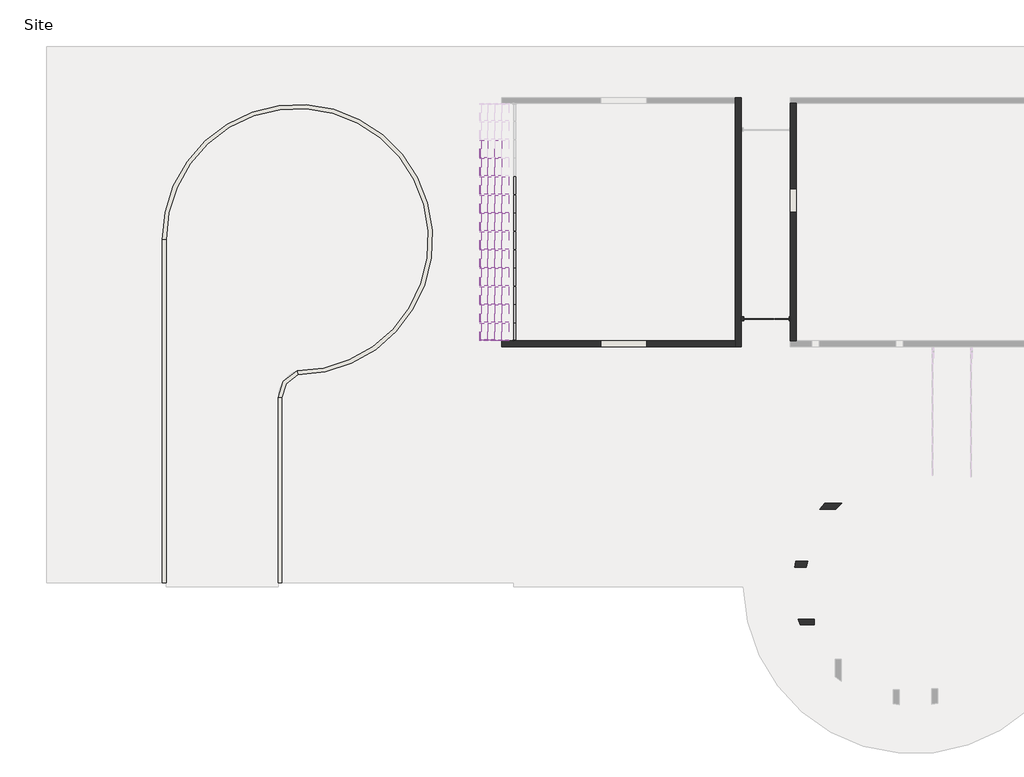
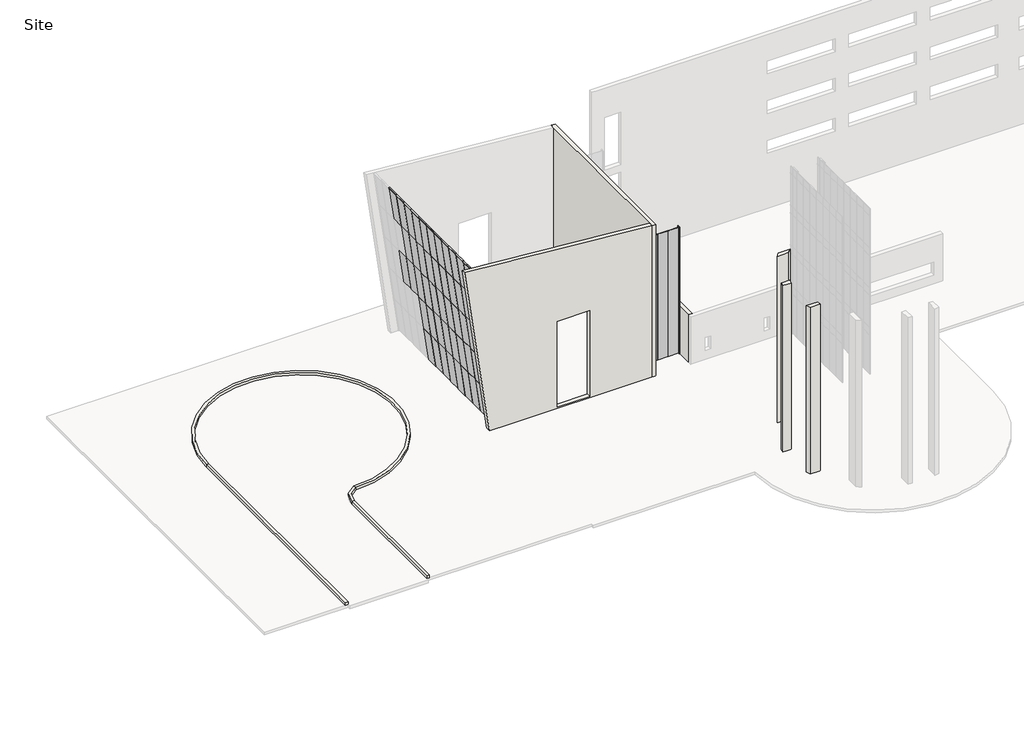
# One storey, part 1 of 4: 53 plates, 16 members, 12 walls.
"""IFC4 building model written with IfcOpenShell, lengths in millimetres."""

import ifcopenshell
import ifcopenshell.guid

model = None  # the IFC model being written
_history = None  # IfcOwnerHistory: only IFC2X3 demands one
_inside = {}  # id of a spatial element -> (the spatial element, [elements in it])
_under = {}  # id of a project, library or spatial element -> (it, [spatial elements below it])
_declared = {}  # id of a project -> (the project, [libraries it declares])
_typed = {}  # id of a type object -> (the type object, [elements of that type])
_made_of = {}  # id of a material, layer set ... -> (it, [elements and type objects made of it])


def new_model(schema):
    """Start an empty IFC model of exactly this schema.

    Asked for "IFC4X3", IfcOpenShell would pick the latest addendum, in which some entities
    have other attributes; the version numbers below select the first issue.
    IFC2X3 requires an IfcOwnerHistory on every rooted entity: one is made here for all.
    """
    global model, _history
    if schema == "IFC4X3":
        model = ifcopenshell.file(schema_version=(4, 3, 0, 0))
    else:
        model = ifcopenshell.file(schema=schema)
    _inside.clear()
    _under.clear()
    _declared.clear()
    _typed.clear()
    _made_of.clear()
    _history = None
    if model.schema == "IFC2X3":
        org = make("IfcOrganization", Name="unknown")
        user = make(
            "IfcPersonAndOrganization",
            ThePerson=make("IfcPerson", FamilyName="unknown"),
            TheOrganization=org,
        )
        app = make(
            "IfcApplication",
            ApplicationDeveloper=org,
            Version="unknown",
            ApplicationFullName="unknown",
            ApplicationIdentifier="unknown",
        )
        _history = make(
            "IfcOwnerHistory",
            OwningUser=user,
            OwningApplication=app,
            ChangeAction="ADDED",
            CreationDate=0,
        )
    return model


def make(cls, **values):
    """One entity of the class cls with the attributes given. An attribute that is None is left unset."""
    return model.create_entity(
        cls, **{name: value for name, value in values.items() if value is not None}
    )


def rooted(cls, **values):
    """An entity with a GlobalId (a new one), such as an element, a storey or a relation."""
    return make(cls, GlobalId=ifcopenshell.guid.new(), OwnerHistory=_history, **values)


def si_unit(unit_type, name, prefix=None):
    """IfcSIUnit, for example si_unit("LENGTHUNIT", "METRE", prefix="MILLI")."""
    return make("IfcSIUnit", UnitType=unit_type, Prefix=prefix, Name=name)


def assignment(units):
    """IfcUnitAssignment: the units of a project."""
    return None if units is None else make("IfcUnitAssignment", Units=units)


def point(xyz):
    """IfcCartesianPoint."""
    return None if xyz is None else make("IfcCartesianPoint", Coordinates=xyz)


def direction(xyz):
    """IfcDirection."""
    return None if xyz is None else make("IfcDirection", DirectionRatios=xyz)


def frame(location, z_axis=None, x_axis=None):
    """IfcAxis2Placement3D, a coordinate frame: its origin and axes. An axis left out is left unset."""
    return make(
        "IfcAxis2Placement3D",
        Location=point(location),
        Axis=direction(z_axis),
        RefDirection=direction(x_axis),
    )


def frame_2d(location, x_axis=None):
    """IfcAxis2Placement2D, a coordinate frame in the plane: its origin and x axis."""
    return make(
        "IfcAxis2Placement2D", Location=point(location), RefDirection=direction(x_axis)
    )


def origin():
    """The frame at (0, 0, 0) with its axes left unset."""
    return frame((0.0, 0.0, 0.0))


def origin_with_axes():
    """The frame at (0, 0, 0) with the z axis (0, 0, 1) and the x axis (1, 0, 0) written out."""
    return frame((0.0, 0.0, 0.0), z_axis=(0.0, 0.0, 1.0), x_axis=(1.0, 0.0, 0.0))


def place(relative_to, where):
    """IfcLocalPlacement: puts the frame where relative to a parent placement (None: the world)."""
    return make(
        "IfcLocalPlacement", PlacementRelTo=relative_to, RelativePlacement=where
    )


def context(
    kind, dimensions, precision=None, world=None, true_north=None, identifier=None
):
    """IfcGeometricRepresentationContext, for example the 3D "Model" context."""
    return make(
        "IfcGeometricRepresentationContext",
        ContextIdentifier=identifier,
        ContextType=kind,
        CoordinateSpaceDimension=dimensions,
        Precision=precision,
        WorldCoordinateSystem=world,
        TrueNorth=true_north,
    )


def project(units=None, contexts=None):
    """IfcProject with its units and contexts."""
    return rooted(
        "IfcProject",
        Name="project",
        RepresentationContexts=contexts,
        UnitsInContext=assignment(units),
    )


def spatial(cls, under=None, at=None, **own):
    """A site, building, storey or space (cls), placed at a placement, below another one or the project."""
    s = rooted(cls, ObjectPlacement=at, **own)
    if under is not None:
        _under.setdefault(under.id(), (under, []))[1].append(s)
    return s


def polyline(points):
    """IfcPolyline through the points."""
    return make("IfcPolyline", Points=[point(p) for p in points])


def circle_curve(where, radius):
    """IfcCircle in the frame where."""
    return make("IfcCircle", Position=where, Radius=radius)


def trimmed(basis, trim1, trim2, sense, master):
    """IfcTrimmedCurve: the piece of a basis curve between two trims."""
    return make(
        "IfcTrimmedCurve",
        BasisCurve=basis,
        Trim1=trim1,
        Trim2=trim2,
        SenseAgreement=sense,
        MasterRepresentation=master,
    )


def segment(curve, same_sense, transition):
    """IfcCompositeCurveSegment."""
    return make(
        "IfcCompositeCurveSegment",
        Transition=transition,
        SameSense=same_sense,
        ParentCurve=curve,
    )


def composite_curve(segments, self_intersect=None):
    """IfcCompositeCurve: segments joined end to end."""
    return make("IfcCompositeCurve", Segments=segments, SelfIntersect=self_intersect)


def outline(outer, holes=None, kind="AREA"):
    """IfcArbitraryClosedProfileDef: a profile drawn as a closed curve; with holes, ...WithVoids."""
    if holes is None:
        return make("IfcArbitraryClosedProfileDef", ProfileType=kind, OuterCurve=outer)
    return make(
        "IfcArbitraryProfileDefWithVoids",
        ProfileType=kind,
        OuterCurve=outer,
        InnerCurves=holes,
    )


def extrude(swept, where, along, depth):
    """IfcExtrudedAreaSolid: the profile swept, set in the frame where, extruded along a direction by depth."""
    return make(
        "IfcExtrudedAreaSolid",
        SweptArea=swept,
        Position=where,
        ExtrudedDirection=direction(along),
        Depth=depth,
    )


def faces_of(points, faces, orient=None, outer=None):
    """IfcFace entities. A face is a list of loops; a loop is a list of indices into points, from 0.

    orient and outer hold one flag for each loop. By default every Orientation is true, the
    first loop of a face is its IfcFaceOuterBound and the others are IfcFaceBound.
    """
    made = []
    for i, loops in enumerate(faces):
        bounds = []
        for j, loop in enumerate(loops):
            is_outer = j == 0 if outer is None else outer[i][j]
            bounds.append(
                make(
                    "IfcFaceOuterBound" if is_outer else "IfcFaceBound",
                    Bound=make("IfcPolyLoop", Polygon=[points[k] for k in loop]),
                    Orientation=True if orient is None else orient[i][j],
                )
            )
        made.append(make("IfcFace", Bounds=bounds))
    return made


def faceted_brep(points, faces, orient=None, outer=None, voids=None):
    """IfcFacetedBrep: a solid bounded by flat faces; with voids (closed shells), ...WithVoids."""
    shared = [point(p) for p in points]
    hull = make("IfcClosedShell", CfsFaces=faces_of(shared, faces, orient, outer))
    if voids is None:
        return make("IfcFacetedBrep", Outer=hull)
    return make(
        "IfcFacetedBrepWithVoids",
        Outer=hull,
        Voids=[
            make(cls, CfsFaces=faces_of(shared, fs, o, b)) for cls, fs, o, b in voids
        ],
    )


def shape(context_of_items, identifier, shape_type, items):
    """IfcShapeRepresentation: the items that make up one representation, for example the "Body"."""
    return make(
        "IfcShapeRepresentation",
        ContextOfItems=context_of_items,
        RepresentationIdentifier=identifier,
        RepresentationType=shape_type,
        Items=items,
    )


def source(mapping_origin, context_of_items, identifier, shape_type, items):
    """IfcRepresentationMap: a shape defined once, which mapped items show again and again."""
    return make(
        "IfcRepresentationMap",
        MappingOrigin=mapping_origin,
        MappedRepresentation=shape(context_of_items, identifier, shape_type, items),
    )


def transform(
    local_origin,
    x_axis=None,
    y_axis=None,
    z_axis=None,
    scale=None,
    scale2=None,
    scale3=None,
    uniform=True,
):
    """IfcCartesianTransformationOperator3D, or its non-uniform kind. x_axis, y_axis, z_axis: its Axis1, 2, 3."""
    if uniform:
        return make(
            "IfcCartesianTransformationOperator3D",
            Axis1=direction(x_axis),
            Axis2=direction(y_axis),
            LocalOrigin=point(local_origin),
            Scale=scale,
            Axis3=direction(z_axis),
        )
    return make(
        "IfcCartesianTransformationOperator3DnonUniform",
        Axis1=direction(x_axis),
        Axis2=direction(y_axis),
        LocalOrigin=point(local_origin),
        Scale=scale,
        Axis3=direction(z_axis),
        Scale2=scale2,
        Scale3=scale3,
    )


def mapped(mapping_source, mapping_target):
    """IfcMappedItem: shows the shape of a source again, moved by a transform."""
    return make(
        "IfcMappedItem", MappingSource=mapping_source, MappingTarget=mapping_target
    )


def made_of(thing, what):
    """Note that an element or type object is made of a material, layer set ...; save() writes the relation."""
    if what is not None:
        _made_of.setdefault(what.id(), (what, []))[1].append(thing)
    return thing


def element(
    cls,
    number,
    at=None,
    inside=None,
    cuts=None,
    type_object=None,
    material=None,
    context=None,
    identifier="Body",
    shape_type=None,
    held_by="IfcProductDefinitionShape",
    body=None,
    shapes=None,
    **own,
):
    """One element of the class cls, such as IfcWall. Its Tag is "e" and its number.

    at: its placement. inside: the storey or other place that contains it. cuts: it is an
    opening in that element (IfcRelVoidsElement). A single representation is given by context,
    identifier, shape_type and body (its items); several are given by shapes. held_by: the class
    of the entity that holds the representations. save() writes the other relations.
    """
    e = rooted(cls, Tag="e%d" % number, ObjectPlacement=at, **own)
    if body is not None:
        shapes = [shape(context, identifier, shape_type, body)]
    if shapes is not None:
        e.Representation = make(held_by, Representations=shapes)
    if inside is not None:
        _inside.setdefault(inside.id(), (inside, []))[1].append(e)
    if cuts is not None:
        rooted(
            "IfcRelVoidsElement", RelatingBuildingElement=cuts, RelatedOpeningElement=e
        )
    if type_object is not None:
        _typed.setdefault(type_object.id(), (type_object, []))[1].append(e)
    return made_of(e, material)


def aggregate(whole, parts):
    """IfcRelAggregates: a whole, such as a stair, and the parts it consists of."""
    return rooted("IfcRelAggregates", RelatingObject=whole, RelatedObjects=parts)


def save(model, path):
    """Write the relations noted so far, then the file.

    IfcRelAggregates (storeys below a building ...), IfcRelContainedInSpatialStructure (elements
    in a storey), IfcRelDefinesByType, IfcRelAssociatesMaterial and IfcRelDeclares: one each for
    every whole, place, type object, material and project.
    """
    for whole, parts in _under.values():
        aggregate(whole, parts)
    for where, things in _inside.values():
        rooted(
            "IfcRelContainedInSpatialStructure",
            RelatedElements=things,
            RelatingStructure=where,
        )
    for kind, things in _typed.values():
        rooted("IfcRelDefinesByType", RelatedObjects=things, RelatingType=kind)
    for what, things in _made_of.values():
        rooted("IfcRelAssociatesMaterial", RelatedObjects=things, RelatingMaterial=what)
    for by, libraries in _declared.values():
        rooted("IfcRelDeclares", RelatingContext=by, RelatedDefinitions=libraries)
    model.write(path)


def member_f8a9089e(model_context):
    return source(origin(), model_context, "Body", "SweptSolid", [
        extrude(outline(polyline([(0.0, 63.5), (0.0, -63.5), (-63.5, -63.5), (-63.5, 63.5), (0.0, 63.5)])), frame((0.0, 0.0, -1320.067308), z_axis=(0.0, 0.0, 1.0), x_axis=(1.0, 0.0, 0.0)), (0.0, 0.0, 1.0), 1320.067308),
    ])


def member_5e02c13a(model_context):
    return source(origin(), model_context, "Body", "SweptSolid", [
        extrude(outline(polyline([(0.0, 63.5), (0.0, -63.5), (-63.5, -63.5), (-63.5, 63.5), (0.0, 63.5)])), frame((0.0, 0.0, -1383.5673076), z_axis=(0.0, 0.0, 1.0), x_axis=(1.0, 0.0, 0.0)), (0.0, 0.0, 1.0), 1383.5673076),
    ])


def member_50cd645d(model_context):
    return source(origin(), model_context, "Body", "SweptSolid", [
        extrude(outline(polyline([(0.0, 63.5), (0.0, -63.5), (-63.5, -63.5), (-63.5, 63.5), (0.0, 63.5)])), frame((0.0, 0.0, -4003.5335741), z_axis=(0.0, 0.0, 1.0), x_axis=(1.0, 0.0, 0.0)), (0.0, 0.0, 1.0), 4003.5335741),
    ])


def member_5d333a65(model_context):
    return source(origin(), model_context, "Body", "SweptSolid", [
        extrude(outline(polyline([(0.0, 63.5), (0.0, -63.5), (-63.5, -63.5), (-63.5, 63.5), (0.0, 63.5)])), frame((0.0, 0.0, -3971.7835741), z_axis=(0.0, 0.0, 1.0), x_axis=(1.0, 0.0, 0.0)), (0.0, 0.0, 1.0), 3971.7835741),
    ])


def system_panel_glazed_21f2c726(model_context):
    return source(origin(), model_context, "Body", "SweptSolid", [
        extrude(outline(polyline([(553.4450969, 19.05), (-553.4450969, 19.05), (-553.4450969, 44.45), (553.4450969, 44.45), (553.4450969, 19.05)])), origin_with_axes(), (0.0, 0.0, 1.0), 14960.6),
    ])


def system_panel_glazed_1400d148(model_context):
    return source(origin(), model_context, "Body", "SweptSolid", [
        extrude(outline(polyline([(569.3200969, 19.05), (-569.3200969, 19.05), (-569.3200969, 44.45), (569.3200969, 44.45), (569.3200969, 19.05)])), origin_with_axes(), (0.0, 0.0, 1.0), 14960.6),
    ])


def system_panel_glazed_f91df05e(model_context):
    return source(origin(), model_context, "Body", "SweptSolid", [
        extrude(outline(polyline([(660.033654, 19.05), (-660.033654, 19.05), (-660.033654, 44.45), (660.033654, 44.45), (660.033654, 19.05)])), origin_with_axes(), (0.0, 0.0, 1.0), 3908.2835741),
    ])


def system_panel_glazed_78b5b18d(model_context):
    return source(origin(), model_context, "Body", "SweptSolid", [
        extrude(outline(polyline([(691.7836538, 19.05), (-691.7836538, 19.05), (-691.7836538, 44.45), (691.7836538, 44.45), (691.7836538, 19.05)])), origin_with_axes(), (0.0, 0.0, 1.0), 3908.2835741),
    ])


model = new_model("IFC4")

# Units and contexts
model_context = context("Model", 3, world=origin())
ifc_project = project(units=[si_unit("LENGTHUNIT", "METRE", prefix="MILLI")], contexts=[model_context])

# Site, building, storey
site = spatial("IfcSite", under=ifc_project)
building = spatial("IfcBuilding", under=site)
storey = spatial("IfcBuildingStorey", under=building, Name="Site", Elevation=-152.4)

# Members
placement = place(None, origin())
member_shape = member_f8a9089e(model_context)
element("IfcMember", 1, ObjectType="Rectangular Mullion1 : 2.5\" x 5\" rectangular", at=placement, inside=storey, context=model_context, shape_type="MappedRepresentation", body=[
    mapped(member_shape, transform((-27908.8595656, 38681.824389, 19574.3667708), x_axis=(-0.13917310096006533, 0.0, 0.9902680687415704), y_axis=(-0.9902680687415704, 0.0, -0.13917310096006533), z_axis=(0.0, -1.0, 0.0))),
])
member_2_shape = member_5e02c13a(model_context)
element("IfcMember", 2, ObjectType="Rectangular Mullion1 : 2.5\" x 5\" rectangular", at=placement, inside=storey, context=model_context, shape_type="MappedRepresentation", body=[
    mapped(member_2_shape, transform((-27908.8595656, 53088.9974658, 19574.3667708), x_axis=(-0.13917310096006533, 0.0, 0.9902680687415704), y_axis=(-0.9902680687415704, 0.0, -0.13917310096006533), z_axis=(0.0, -1.0, 0.0))),
])
element("IfcMember", 3, ObjectType="Rectangular Mullion1 : 2.5\" x 5\" rectangular", at=placement, inside=storey, context=model_context, shape_type="MappedRepresentation", body=[
    mapped(member_2_shape, transform((-27908.8595656, 51641.9301581, 19574.3667708), x_axis=(-0.13917310096006533, 0.0, 0.9902680687415704), y_axis=(-0.9902680687415704, 0.0, -0.13917310096006533), z_axis=(0.0, -1.0, 0.0))),
])
element("IfcMember", 4, ObjectType="Rectangular Mullion1 : 2.5\" x 5\" rectangular", at=placement, inside=storey, context=model_context, shape_type="MappedRepresentation", body=[
    mapped(member_2_shape, transform((-27908.8595656, 50194.8628505, 19574.3667708), x_axis=(-0.13917310096006533, 0.0, 0.9902680687415704), y_axis=(-0.9902680687415704, 0.0, -0.13917310096006533), z_axis=(0.0, -1.0, 0.0))),
])
element("IfcMember", 5, ObjectType="Rectangular Mullion1 : 2.5\" x 5\" rectangular", at=placement, inside=storey, context=model_context, shape_type="MappedRepresentation", body=[
    mapped(member_2_shape, transform((-27908.8595656, 48747.7955428, 19574.3667708), x_axis=(-0.13917310096006533, 0.0, 0.9902680687415704), y_axis=(-0.9902680687415704, 0.0, -0.13917310096006533), z_axis=(0.0, -1.0, 0.0))),
])
element("IfcMember", 6, ObjectType="Rectangular Mullion1 : 2.5\" x 5\" rectangular", at=placement, inside=storey, context=model_context, shape_type="MappedRepresentation", body=[
    mapped(member_2_shape, transform((-27908.8595656, 47300.7282352, 19574.3667708), x_axis=(-0.13917310096006533, 0.0, 0.9902680687415704), y_axis=(-0.9902680687415704, 0.0, -0.13917310096006533), z_axis=(0.0, -1.0, 0.0))),
])
element("IfcMember", 7, ObjectType="Rectangular Mullion1 : 2.5\" x 5\" rectangular", at=placement, inside=storey, context=model_context, shape_type="MappedRepresentation", body=[
    mapped(member_2_shape, transform((-27908.8595656, 45853.6609275, 19574.3667708), x_axis=(-0.13917310096006533, 0.0, 0.9902680687415704), y_axis=(-0.9902680687415704, 0.0, -0.13917310096006533), z_axis=(0.0, -1.0, 0.0))),
])
element("IfcMember", 8, ObjectType="Rectangular Mullion1 : 2.5\" x 5\" rectangular", at=placement, inside=storey, context=model_context, shape_type="MappedRepresentation", body=[
    mapped(member_2_shape, transform((-27908.8595656, 44406.5936199, 19574.3667708), x_axis=(-0.13917310096006533, 0.0, 0.9902680687415704), y_axis=(-0.9902680687415704, 0.0, -0.13917310096006533), z_axis=(0.0, -1.0, 0.0))),
])
element("IfcMember", 9, ObjectType="Rectangular Mullion1 : 2.5\" x 5\" rectangular", at=placement, inside=storey, context=model_context, shape_type="MappedRepresentation", body=[
    mapped(member_2_shape, transform((-27908.8595656, 42959.5263122, 19574.3667708), x_axis=(-0.13917310096006533, 0.0, 0.9902680687415704), y_axis=(-0.9902680687415704, 0.0, -0.13917310096006533), z_axis=(0.0, -1.0, 0.0))),
])
element("IfcMember", 10, ObjectType="Rectangular Mullion1 : 2.5\" x 5\" rectangular", at=placement, inside=storey, context=model_context, shape_type="MappedRepresentation", body=[
    mapped(member_2_shape, transform((-27908.8595656, 41512.4590046, 19574.3667708), x_axis=(-0.13917310096006533, 0.0, 0.9902680687415704), y_axis=(-0.9902680687415704, 0.0, -0.13917310096006533), z_axis=(0.0, -1.0, 0.0))),
])
element("IfcMember", 11, ObjectType="Rectangular Mullion1 : 2.5\" x 5\" rectangular", at=placement, inside=storey, context=model_context, shape_type="MappedRepresentation", body=[
    mapped(member_2_shape, transform((-27908.8595656, 40065.391697, 19574.3667708), x_axis=(-0.13917310096006533, 0.0, 0.9902680687415704), y_axis=(-0.9902680687415704, 0.0, -0.13917310096006533), z_axis=(0.0, -1.0, 0.0))),
])
member_3_shape = member_50cd645d(model_context)
element("IfcMember", 12, ObjectType="Rectangular Mullion1 : 2.5\" x 5\" rectangular", at=placement, inside=storey, context=model_context, shape_type="MappedRepresentation", body=[
    mapped(member_3_shape, transform((-25136.1948919, 38618.324389, -154.1674984), x_axis=(0.0, -1.0, 0.0), y_axis=(-0.99026806874157, 0.0, -0.1391731009600678), z_axis=(0.1391731009600678, 0.0, -0.99026806874157))),
])
member_4_shape = member_5d333a65(model_context)
element("IfcMember", 13, ObjectType="Rectangular Mullion1 : 2.5\" x 5\" rectangular", at=placement, inside=storey, context=model_context, shape_type="MappedRepresentation", body=[
    mapped(member_4_shape, transform((-25693.3790742, 38618.324389, 3810.4039622), x_axis=(0.0, -1.0, 0.0), y_axis=(-0.9902680687415704, 0.0, -0.13917310096006566), z_axis=(0.13917310096006566, 0.0, -0.9902680687415704))),
])
element("IfcMember", 14, ObjectType="Rectangular Mullion1 : 2.5\" x 5\" rectangular", at=placement, inside=storey, context=model_context, shape_type="MappedRepresentation", body=[
    mapped(member_4_shape, transform((-26246.1445106, 38618.324389, 7743.5344115), x_axis=(0.0, -1.0, 0.0), y_axis=(-0.9902680687415704, 0.0, -0.13917310096006574), z_axis=(0.13917310096006574, 0.0, -0.9902680687415704))),
])
element("IfcMember", 15, ObjectType="Rectangular Mullion1 : 2.5\" x 5\" rectangular", at=placement, inside=storey, context=model_context, shape_type="MappedRepresentation", body=[
    mapped(member_4_shape, transform((-26798.9099469, 38618.324389, 11676.6648609), x_axis=(0.0, -1.0, 0.0), y_axis=(-0.9902680687415705, 0.0, -0.13917310096006458), z_axis=(0.13917310096006458, 0.0, -0.9902680687415705))),
])
element("IfcMember", 16, ObjectType="Rectangular Mullion1 : 2.5\" x 5\" rectangular", at=placement, inside=storey, context=model_context, shape_type="MappedRepresentation", body=[
    mapped(member_3_shape, transform((-27351.6753833, 38618.324389, 15609.7953102), x_axis=(0.0, -1.0, 0.0), y_axis=(-0.9902680687415704, 0.0, -0.13917310096006558), z_axis=(0.13917310096006558, 0.0, -0.9902680687415704))),
])

# Plates
system_panel_glazed_shape = system_panel_glazed_21f2c726(model_context)
element("IfcPlate", 17, ObjectType="System Panel : Glazed", at=placement, inside=storey, context=model_context, shape_type="MappedRepresentation", body=[
    mapped(system_panel_glazed_shape, transform((-4114.5553134, 40372.511889, -88.9), x_axis=(-1.0, 0.0, 0.0), y_axis=(0.0, -1.0, 0.0), z_axis=(0.0, 0.0, 1.0))),
])
element("IfcPlate", 18, ObjectType="System Panel : Glazed", at=placement, inside=storey, context=model_context, shape_type="MappedRepresentation", body=[
    mapped(system_panel_glazed_shape, transform((-6487.0857008, 40372.511889, -88.9), x_axis=(-1.0, 0.0, 0.0), y_axis=(0.0, -1.0, 0.0), z_axis=(0.0, 0.0, 1.0))),
])
system_panel_glazed_2_shape = system_panel_glazed_1400d148(model_context)
element("IfcPlate", 19, ObjectType="System Panel : Glazed", at=placement, inside=storey, context=model_context, shape_type="MappedRepresentation", body=[
    mapped(system_panel_glazed_2_shape, transform((-5300.8205071, 40372.511889, -88.9), x_axis=(-1.0, 0.0, 0.0), y_axis=(0.0, -1.0, 0.0), z_axis=(0.0, 0.0, 1.0))),
])
system_panel_glazed_3_shape = system_panel_glazed_f91df05e(model_context)
element("IfcPlate", 20, ObjectType="System Panel : Glazed", at=placement, inside=storey, context=model_context, shape_type="MappedRepresentation", body=[
    mapped(system_panel_glazed_3_shape, transform((-25145.0323838, 39341.858043, -91.285476), x_axis=(0.0, -1.0, 0.0), y_axis=(0.9902680687415704, 0.0, 0.13917310096006547), z_axis=(-0.13917310096006547, 0.0, 0.9902680687415704))),
])
element("IfcPlate", 21, ObjectType="System Panel : Glazed", at=placement, inside=storey, context=model_context, shape_type="MappedRepresentation", body=[
    mapped(system_panel_glazed_3_shape, transform((-25697.7978202, 39341.858043, 3841.8449733), x_axis=(0.0, -1.0, 0.0), y_axis=(0.9902680687415704, 0.0, 0.13917310096006533), z_axis=(-0.13917310096006533, 0.0, 0.9902680687415704))),
])
element("IfcPlate", 22, ObjectType="System Panel : Glazed", at=placement, inside=storey, context=model_context, shape_type="MappedRepresentation", body=[
    mapped(system_panel_glazed_3_shape, transform((-26250.5632565, 39341.858043, 7774.9754227), x_axis=(0.0, -1.0, 0.0), y_axis=(0.9902680687415704, 0.0, 0.13917310096006533), z_axis=(-0.13917310096006533, 0.0, 0.9902680687415704))),
])
element("IfcPlate", 23, ObjectType="System Panel : Glazed", at=placement, inside=storey, context=model_context, shape_type="MappedRepresentation", body=[
    mapped(system_panel_glazed_3_shape, transform((-26803.3286929, 39341.858043, 11708.105872), x_axis=(0.0, -1.0, 0.0), y_axis=(0.9902680687415704, 0.0, 0.13917310096006533), z_axis=(-0.13917310096006533, 0.0, 0.9902680687415704))),
])
element("IfcPlate", 24, ObjectType="System Panel : Glazed", at=placement, inside=storey, context=model_context, shape_type="MappedRepresentation", body=[
    mapped(system_panel_glazed_3_shape, transform((-27356.0941292, 39341.858043, 15641.2363214), x_axis=(0.0, -1.0, 0.0), y_axis=(0.9902680687415704, 0.0, 0.13917310096006533), z_axis=(-0.13917310096006533, 0.0, 0.9902680687415704))),
])
system_panel_glazed_4_shape = system_panel_glazed_78b5b18d(model_context)
element("IfcPlate", 25, ObjectType="System Panel : Glazed", at=placement, inside=storey, context=model_context, shape_type="MappedRepresentation", body=[
    mapped(system_panel_glazed_4_shape, transform((-25145.0323838, 50886.6465043, -91.285476), x_axis=(0.0, -1.0, 0.0), y_axis=(0.9902680687415704, 0.0, 0.13917310096006547), z_axis=(-0.13917310096006547, 0.0, 0.9902680687415704))),
])
element("IfcPlate", 26, ObjectType="System Panel : Glazed", at=placement, inside=storey, context=model_context, shape_type="MappedRepresentation", body=[
    mapped(system_panel_glazed_4_shape, transform((-25145.0323838, 49439.5791967, -91.285476), x_axis=(0.0, -1.0, 0.0), y_axis=(0.9902680687415704, 0.0, 0.13917310096006547), z_axis=(-0.13917310096006547, 0.0, 0.9902680687415704))),
])
element("IfcPlate", 27, ObjectType="System Panel : Glazed", at=placement, inside=storey, context=model_context, shape_type="MappedRepresentation", body=[
    mapped(system_panel_glazed_4_shape, transform((-25145.0323838, 47992.511889, -91.285476), x_axis=(0.0, -1.0, 0.0), y_axis=(0.9902680687415704, 0.0, 0.13917310096006547), z_axis=(-0.13917310096006547, 0.0, 0.9902680687415704))),
])
element("IfcPlate", 28, ObjectType="System Panel : Glazed", at=placement, inside=storey, context=model_context, shape_type="MappedRepresentation", body=[
    mapped(system_panel_glazed_4_shape, transform((-25145.0323838, 46545.4445814, -91.285476), x_axis=(0.0, -1.0, 0.0), y_axis=(0.9902680687415704, 0.0, 0.13917310096006547), z_axis=(-0.13917310096006547, 0.0, 0.9902680687415704))),
])
element("IfcPlate", 29, ObjectType="System Panel : Glazed", at=placement, inside=storey, context=model_context, shape_type="MappedRepresentation", body=[
    mapped(system_panel_glazed_4_shape, transform((-25145.0323838, 45098.3772737, -91.285476), x_axis=(0.0, -1.0, 0.0), y_axis=(0.9902680687415704, 0.0, 0.13917310096006547), z_axis=(-0.13917310096006547, 0.0, 0.9902680687415704))),
])
element("IfcPlate", 30, ObjectType="System Panel : Glazed", at=placement, inside=storey, context=model_context, shape_type="MappedRepresentation", body=[
    mapped(system_panel_glazed_4_shape, transform((-25145.0323838, 43651.3099661, -91.285476), x_axis=(0.0, -1.0, 0.0), y_axis=(0.9902680687415704, 0.0, 0.13917310096006547), z_axis=(-0.13917310096006547, 0.0, 0.9902680687415704))),
])
element("IfcPlate", 31, ObjectType="System Panel : Glazed", at=placement, inside=storey, context=model_context, shape_type="MappedRepresentation", body=[
    mapped(system_panel_glazed_4_shape, transform((-25145.0323838, 42204.2426584, -91.285476), x_axis=(0.0, -1.0, 0.0), y_axis=(0.9902680687415704, 0.0, 0.13917310096006547), z_axis=(-0.13917310096006547, 0.0, 0.9902680687415704))),
])
element("IfcPlate", 32, ObjectType="System Panel : Glazed", at=placement, inside=storey, context=model_context, shape_type="MappedRepresentation", body=[
    mapped(system_panel_glazed_4_shape, transform((-25145.0323838, 40757.1753508, -91.285476), x_axis=(0.0, -1.0, 0.0), y_axis=(0.9902680687415704, 0.0, 0.13917310096006547), z_axis=(-0.13917310096006547, 0.0, 0.9902680687415704))),
])
element("IfcPlate", 33, ObjectType="System Panel : Glazed", at=placement, inside=storey, context=model_context, shape_type="MappedRepresentation", body=[
    mapped(system_panel_glazed_4_shape, transform((-25697.7978202, 50886.6465043, 3841.8449733), x_axis=(0.0, -1.0, 0.0), y_axis=(0.9902680687415704, 0.0, 0.13917310096006533), z_axis=(-0.13917310096006533, 0.0, 0.9902680687415704))),
])
element("IfcPlate", 34, ObjectType="System Panel : Glazed", at=placement, inside=storey, context=model_context, shape_type="MappedRepresentation", body=[
    mapped(system_panel_glazed_4_shape, transform((-25697.7978202, 49439.5791967, 3841.8449733), x_axis=(0.0, -1.0, 0.0), y_axis=(0.9902680687415704, 0.0, 0.13917310096006533), z_axis=(-0.13917310096006533, 0.0, 0.9902680687415704))),
])
element("IfcPlate", 35, ObjectType="System Panel : Glazed", at=placement, inside=storey, context=model_context, shape_type="MappedRepresentation", body=[
    mapped(system_panel_glazed_4_shape, transform((-25697.7978202, 47992.511889, 3841.8449733), x_axis=(0.0, -1.0, 0.0), y_axis=(0.9902680687415704, 0.0, 0.13917310096006533), z_axis=(-0.13917310096006533, 0.0, 0.9902680687415704))),
])
element("IfcPlate", 36, ObjectType="System Panel : Glazed", at=placement, inside=storey, context=model_context, shape_type="MappedRepresentation", body=[
    mapped(system_panel_glazed_4_shape, transform((-25697.7978202, 46545.4445814, 3841.8449733), x_axis=(0.0, -1.0, 0.0), y_axis=(0.9902680687415704, 0.0, 0.13917310096006533), z_axis=(-0.13917310096006533, 0.0, 0.9902680687415704))),
])
element("IfcPlate", 37, ObjectType="System Panel : Glazed", at=placement, inside=storey, context=model_context, shape_type="MappedRepresentation", body=[
    mapped(system_panel_glazed_4_shape, transform((-25697.7978202, 45098.3772737, 3841.8449733), x_axis=(0.0, -1.0, 0.0), y_axis=(0.9902680687415704, 0.0, 0.13917310096006533), z_axis=(-0.13917310096006533, 0.0, 0.9902680687415704))),
])
element("IfcPlate", 38, ObjectType="System Panel : Glazed", at=placement, inside=storey, context=model_context, shape_type="MappedRepresentation", body=[
    mapped(system_panel_glazed_4_shape, transform((-25697.7978202, 43651.3099661, 3841.8449733), x_axis=(0.0, -1.0, 0.0), y_axis=(0.9902680687415704, 0.0, 0.13917310096006533), z_axis=(-0.13917310096006533, 0.0, 0.9902680687415704))),
])
element("IfcPlate", 39, ObjectType="System Panel : Glazed", at=placement, inside=storey, context=model_context, shape_type="MappedRepresentation", body=[
    mapped(system_panel_glazed_4_shape, transform((-25697.7978202, 42204.2426584, 3841.8449733), x_axis=(0.0, -1.0, 0.0), y_axis=(0.9902680687415704, 0.0, 0.13917310096006533), z_axis=(-0.13917310096006533, 0.0, 0.9902680687415704))),
])
element("IfcPlate", 40, ObjectType="System Panel : Glazed", at=placement, inside=storey, context=model_context, shape_type="MappedRepresentation", body=[
    mapped(system_panel_glazed_4_shape, transform((-25697.7978202, 40757.1753508, 3841.8449733), x_axis=(0.0, -1.0, 0.0), y_axis=(0.9902680687415704, 0.0, 0.13917310096006533), z_axis=(-0.13917310096006533, 0.0, 0.9902680687415704))),
])
element("IfcPlate", 41, ObjectType="System Panel : Glazed", at=placement, inside=storey, context=model_context, shape_type="MappedRepresentation", body=[
    mapped(system_panel_glazed_4_shape, transform((-26250.5632565, 53780.7811196, 7774.9754227), x_axis=(0.0, -1.0, 0.0), y_axis=(0.9902680687415704, 0.0, 0.13917310096006533), z_axis=(-0.13917310096006533, 0.0, 0.9902680687415704))),
])
element("IfcPlate", 42, ObjectType="System Panel : Glazed", at=placement, inside=storey, context=model_context, shape_type="MappedRepresentation", body=[
    mapped(system_panel_glazed_4_shape, transform((-26250.5632565, 52333.7138119, 7774.9754227), x_axis=(0.0, -1.0, 0.0), y_axis=(0.9902680687415704, 0.0, 0.13917310096006533), z_axis=(-0.13917310096006533, 0.0, 0.9902680687415704))),
])
element("IfcPlate", 43, ObjectType="System Panel : Glazed", at=placement, inside=storey, context=model_context, shape_type="MappedRepresentation", body=[
    mapped(system_panel_glazed_4_shape, transform((-26250.5632565, 50886.6465043, 7774.9754227), x_axis=(0.0, -1.0, 0.0), y_axis=(0.9902680687415704, 0.0, 0.13917310096006533), z_axis=(-0.13917310096006533, 0.0, 0.9902680687415704))),
])
element("IfcPlate", 44, ObjectType="System Panel : Glazed", at=placement, inside=storey, context=model_context, shape_type="MappedRepresentation", body=[
    mapped(system_panel_glazed_4_shape, transform((-26250.5632565, 49439.5791967, 7774.9754227), x_axis=(0.0, -1.0, 0.0), y_axis=(0.9902680687415704, 0.0, 0.13917310096006533), z_axis=(-0.13917310096006533, 0.0, 0.9902680687415704))),
])
element("IfcPlate", 45, ObjectType="System Panel : Glazed", at=placement, inside=storey, context=model_context, shape_type="MappedRepresentation", body=[
    mapped(system_panel_glazed_4_shape, transform((-26250.5632565, 47992.511889, 7774.9754227), x_axis=(0.0, -1.0, 0.0), y_axis=(0.9902680687415704, 0.0, 0.13917310096006533), z_axis=(-0.13917310096006533, 0.0, 0.9902680687415704))),
])
element("IfcPlate", 46, ObjectType="System Panel : Glazed", at=placement, inside=storey, context=model_context, shape_type="MappedRepresentation", body=[
    mapped(system_panel_glazed_4_shape, transform((-26250.5632565, 46545.4445814, 7774.9754227), x_axis=(0.0, -1.0, 0.0), y_axis=(0.9902680687415704, 0.0, 0.13917310096006533), z_axis=(-0.13917310096006533, 0.0, 0.9902680687415704))),
])
element("IfcPlate", 47, ObjectType="System Panel : Glazed", at=placement, inside=storey, context=model_context, shape_type="MappedRepresentation", body=[
    mapped(system_panel_glazed_4_shape, transform((-26250.5632565, 45098.3772737, 7774.9754227), x_axis=(0.0, -1.0, 0.0), y_axis=(0.9902680687415704, 0.0, 0.13917310096006533), z_axis=(-0.13917310096006533, 0.0, 0.9902680687415704))),
])
element("IfcPlate", 48, ObjectType="System Panel : Glazed", at=placement, inside=storey, context=model_context, shape_type="MappedRepresentation", body=[
    mapped(system_panel_glazed_4_shape, transform((-26250.5632565, 43651.3099661, 7774.9754227), x_axis=(0.0, -1.0, 0.0), y_axis=(0.9902680687415704, 0.0, 0.13917310096006533), z_axis=(-0.13917310096006533, 0.0, 0.9902680687415704))),
])
element("IfcPlate", 49, ObjectType="System Panel : Glazed", at=placement, inside=storey, context=model_context, shape_type="MappedRepresentation", body=[
    mapped(system_panel_glazed_4_shape, transform((-26250.5632565, 42204.2426584, 7774.9754227), x_axis=(0.0, -1.0, 0.0), y_axis=(0.9902680687415704, 0.0, 0.13917310096006533), z_axis=(-0.13917310096006533, 0.0, 0.9902680687415704))),
])
element("IfcPlate", 50, ObjectType="System Panel : Glazed", at=placement, inside=storey, context=model_context, shape_type="MappedRepresentation", body=[
    mapped(system_panel_glazed_4_shape, transform((-26250.5632565, 40757.1753508, 7774.9754227), x_axis=(0.0, -1.0, 0.0), y_axis=(0.9902680687415704, 0.0, 0.13917310096006533), z_axis=(-0.13917310096006533, 0.0, 0.9902680687415704))),
])
element("IfcPlate", 51, ObjectType="System Panel : Glazed", at=placement, inside=storey, context=model_context, shape_type="MappedRepresentation", body=[
    mapped(system_panel_glazed_4_shape, transform((-26803.3286929, 52333.7138119, 11708.105872), x_axis=(0.0, -1.0, 0.0), y_axis=(0.9902680687415704, 0.0, 0.13917310096006533), z_axis=(-0.13917310096006533, 0.0, 0.9902680687415704))),
])
element("IfcPlate", 52, ObjectType="System Panel : Glazed", at=placement, inside=storey, context=model_context, shape_type="MappedRepresentation", body=[
    mapped(system_panel_glazed_4_shape, transform((-26803.3286929, 50886.6465043, 11708.105872), x_axis=(0.0, -1.0, 0.0), y_axis=(0.9902680687415704, 0.0, 0.13917310096006533), z_axis=(-0.13917310096006533, 0.0, 0.9902680687415704))),
])
element("IfcPlate", 53, ObjectType="System Panel : Glazed", at=placement, inside=storey, context=model_context, shape_type="MappedRepresentation", body=[
    mapped(system_panel_glazed_4_shape, transform((-26803.3286929, 49439.5791967, 11708.105872), x_axis=(0.0, -1.0, 0.0), y_axis=(0.9902680687415704, 0.0, 0.13917310096006533), z_axis=(-0.13917310096006533, 0.0, 0.9902680687415704))),
])
element("IfcPlate", 54, ObjectType="System Panel : Glazed", at=placement, inside=storey, context=model_context, shape_type="MappedRepresentation", body=[
    mapped(system_panel_glazed_4_shape, transform((-26803.3286929, 47992.511889, 11708.105872), x_axis=(0.0, -1.0, 0.0), y_axis=(0.9902680687415704, 0.0, 0.13917310096006533), z_axis=(-0.13917310096006533, 0.0, 0.9902680687415704))),
])
element("IfcPlate", 55, ObjectType="System Panel : Glazed", at=placement, inside=storey, context=model_context, shape_type="MappedRepresentation", body=[
    mapped(system_panel_glazed_4_shape, transform((-26803.3286929, 46545.4445814, 11708.105872), x_axis=(0.0, -1.0, 0.0), y_axis=(0.9902680687415704, 0.0, 0.13917310096006533), z_axis=(-0.13917310096006533, 0.0, 0.9902680687415704))),
])
element("IfcPlate", 56, ObjectType="System Panel : Glazed", at=placement, inside=storey, context=model_context, shape_type="MappedRepresentation", body=[
    mapped(system_panel_glazed_4_shape, transform((-26803.3286929, 45098.3772737, 11708.105872), x_axis=(0.0, -1.0, 0.0), y_axis=(0.9902680687415704, 0.0, 0.13917310096006533), z_axis=(-0.13917310096006533, 0.0, 0.9902680687415704))),
])
element("IfcPlate", 57, ObjectType="System Panel : Glazed", at=placement, inside=storey, context=model_context, shape_type="MappedRepresentation", body=[
    mapped(system_panel_glazed_4_shape, transform((-26803.3286929, 43651.3099661, 11708.105872), x_axis=(0.0, -1.0, 0.0), y_axis=(0.9902680687415704, 0.0, 0.13917310096006533), z_axis=(-0.13917310096006533, 0.0, 0.9902680687415704))),
])
element("IfcPlate", 58, ObjectType="System Panel : Glazed", at=placement, inside=storey, context=model_context, shape_type="MappedRepresentation", body=[
    mapped(system_panel_glazed_4_shape, transform((-26803.3286929, 42204.2426584, 11708.105872), x_axis=(0.0, -1.0, 0.0), y_axis=(0.9902680687415704, 0.0, 0.13917310096006533), z_axis=(-0.13917310096006533, 0.0, 0.9902680687415704))),
])
element("IfcPlate", 59, ObjectType="System Panel : Glazed", at=placement, inside=storey, context=model_context, shape_type="MappedRepresentation", body=[
    mapped(system_panel_glazed_4_shape, transform((-26803.3286929, 40757.1753508, 11708.105872), x_axis=(0.0, -1.0, 0.0), y_axis=(0.9902680687415704, 0.0, 0.13917310096006533), z_axis=(-0.13917310096006533, 0.0, 0.9902680687415704))),
])
element("IfcPlate", 60, ObjectType="System Panel : Glazed", at=placement, inside=storey, context=model_context, shape_type="MappedRepresentation", body=[
    mapped(system_panel_glazed_4_shape, transform((-27356.0941292, 53780.7811196, 15641.2363214), x_axis=(0.0, -1.0, 0.0), y_axis=(0.9902680687415704, 0.0, 0.13917310096006533), z_axis=(-0.13917310096006533, 0.0, 0.9902680687415704))),
])
element("IfcPlate", 61, ObjectType="System Panel : Glazed", at=placement, inside=storey, context=model_context, shape_type="MappedRepresentation", body=[
    mapped(system_panel_glazed_4_shape, transform((-27356.0941292, 52333.7138119, 15641.2363214), x_axis=(0.0, -1.0, 0.0), y_axis=(0.9902680687415704, 0.0, 0.13917310096006533), z_axis=(-0.13917310096006533, 0.0, 0.9902680687415704))),
])
element("IfcPlate", 62, ObjectType="System Panel : Glazed", at=placement, inside=storey, context=model_context, shape_type="MappedRepresentation", body=[
    mapped(system_panel_glazed_4_shape, transform((-27356.0941292, 50886.6465043, 15641.2363214), x_axis=(0.0, -1.0, 0.0), y_axis=(0.9902680687415704, 0.0, 0.13917310096006533), z_axis=(-0.13917310096006533, 0.0, 0.9902680687415704))),
])
element("IfcPlate", 63, ObjectType="System Panel : Glazed", at=placement, inside=storey, context=model_context, shape_type="MappedRepresentation", body=[
    mapped(system_panel_glazed_4_shape, transform((-27356.0941292, 49439.5791967, 15641.2363214), x_axis=(0.0, -1.0, 0.0), y_axis=(0.9902680687415704, 0.0, 0.13917310096006533), z_axis=(-0.13917310096006533, 0.0, 0.9902680687415704))),
])
element("IfcPlate", 64, ObjectType="System Panel : Glazed", at=placement, inside=storey, context=model_context, shape_type="MappedRepresentation", body=[
    mapped(system_panel_glazed_4_shape, transform((-27356.0941292, 47992.511889, 15641.2363214), x_axis=(0.0, -1.0, 0.0), y_axis=(0.9902680687415704, 0.0, 0.13917310096006533), z_axis=(-0.13917310096006533, 0.0, 0.9902680687415704))),
])
element("IfcPlate", 65, ObjectType="System Panel : Glazed", at=placement, inside=storey, context=model_context, shape_type="MappedRepresentation", body=[
    mapped(system_panel_glazed_4_shape, transform((-27356.0941292, 46545.4445814, 15641.2363214), x_axis=(0.0, -1.0, 0.0), y_axis=(0.9902680687415704, 0.0, 0.13917310096006533), z_axis=(-0.13917310096006533, 0.0, 0.9902680687415704))),
])
element("IfcPlate", 66, ObjectType="System Panel : Glazed", at=placement, inside=storey, context=model_context, shape_type="MappedRepresentation", body=[
    mapped(system_panel_glazed_4_shape, transform((-27356.0941292, 45098.3772737, 15641.2363214), x_axis=(0.0, -1.0, 0.0), y_axis=(0.9902680687415704, 0.0, 0.13917310096006533), z_axis=(-0.13917310096006533, 0.0, 0.9902680687415704))),
])
element("IfcPlate", 67, ObjectType="System Panel : Glazed", at=placement, inside=storey, context=model_context, shape_type="MappedRepresentation", body=[
    mapped(system_panel_glazed_4_shape, transform((-27356.0941292, 43651.3099661, 15641.2363214), x_axis=(0.0, -1.0, 0.0), y_axis=(0.9902680687415704, 0.0, 0.13917310096006533), z_axis=(-0.13917310096006533, 0.0, 0.9902680687415704))),
])
element("IfcPlate", 68, ObjectType="System Panel : Glazed", at=placement, inside=storey, context=model_context, shape_type="MappedRepresentation", body=[
    mapped(system_panel_glazed_4_shape, transform((-27356.0941292, 42204.2426584, 15641.2363214), x_axis=(0.0, -1.0, 0.0), y_axis=(0.9902680687415704, 0.0, 0.13917310096006533), z_axis=(-0.13917310096006533, 0.0, 0.9902680687415704))),
])
element("IfcPlate", 69, ObjectType="System Panel : Glazed", at=placement, inside=storey, context=model_context, shape_type="MappedRepresentation", body=[
    mapped(system_panel_glazed_4_shape, transform((-27356.0941292, 40757.1753508, 15641.2363214), x_axis=(0.0, -1.0, 0.0), y_axis=(0.9902680687415704, 0.0, 0.13917310096006533), z_axis=(-0.13917310096006533, 0.0, 0.9902680687415704))),
])

# Walls
element("IfcWall", 70, ObjectType="Generic - 12\"", at=placement, inside=storey, context=model_context, shape_type="SweptSolid", body=[
    extrude(outline(polyline([(-52722.4307976, 46620.911889), (-52722.4307976, 19493.711889), (-53027.2307976, 19493.711889), (-53027.2307976, 46620.911889), (-52722.4307976, 46620.911889)])), frame((0.0, 0.0, -152.4), z_axis=(0.0, 0.0, 1.0), x_axis=(1.0, 0.0, 0.0)), (0.0, 0.0, 1.0), 304.8),
])
element("IfcWall", 71, ObjectType="Generic - 12\"", at=placement, inside=storey, context=model_context, shape_type="SweptSolid", body=[
    extrude(outline(composite_curve([segment(polyline([(-42332.6379779, 35952.9450339), (-42384.6461103, 36257.743054)]), True, "CONTINUOUS"), segment(trimmed(circle_curve(frame_2d((-42359.2307976, 46620.911889)), 10363.2), [point((-42384.6461103, 36257.743054))], [point((-52722.4307976, 46620.911889))], True, "CARTESIAN"), True, "CONTINUOUS"), segment(polyline([(-52722.4307976, 46620.911889), (-53027.2307976, 46620.911889)]), True, "CONTINUOUS"), segment(trimmed(circle_curve(frame_2d((-42359.2307976, 46620.911889)), 10668.0), [point((-53027.2307976, 46620.911889))], [point((-42332.6379779, 35952.9450339))], False, "CARTESIAN"), True, "CONTINUOUS")], self_intersect=False)), frame((0.0, 0.0, -152.4), z_axis=(0.0, 0.0, 1.0), x_axis=(1.0, 0.0, 0.0)), (0.0, 0.0, 1.0), 304.8),
])
element("IfcWall", 72, ObjectType="Generic - 12\"", at=placement, inside=storey, context=model_context, shape_type="SweptSolid", body=[
    extrude(outline(polyline([(-43578.4307976, 34125.8154666), (-43578.4307976, 19493.711889), (-43883.2307976, 19493.711889), (-43883.2307976, 34122.4704857), (-43578.4307976, 34125.8154666)])), frame((0.0, 0.0, -152.4), z_axis=(0.0, 0.0, 1.0), x_axis=(1.0, 0.0, 0.0)), (0.0, 0.0, 1.0), 304.8),
])
element("IfcWall", 73, ObjectType="Generic - 12\"", at=placement, inside=storey, context=model_context, shape_type="SweptSolid", body=[
    extrude(outline(composite_curve([segment(polyline([(-43578.4307976, 34125.8154666), (-43883.2307976, 34122.4704857)]), True, "CONTINUOUS"), segment(trimmed(circle_curve(frame_2d((-41679.1721267, 34169.1174245)), 2204.5522361), [point((-43883.2307976, 34122.4704857))], [point((-42384.6461103, 36257.743054))], False, "CARTESIAN"), True, "CONTINUOUS"), segment(polyline([(-42384.6461103, 36257.743054), (-42332.6379779, 35952.9450339)]), True, "CONTINUOUS"), segment(trimmed(circle_curve(frame_2d((-41679.1721267, 34169.1174245)), 1899.7522361), [point((-42332.6379779, 35952.9450339))], [point((-43578.4307976, 34125.8154666))], True, "CARTESIAN"), True, "CONTINUOUS")], self_intersect=False)), frame((0.0, 0.0, -152.4), z_axis=(0.0, 0.0, 1.0), x_axis=(1.0, 0.0, 0.0)), (0.0, 0.0, 1.0), 304.8),
])
element("IfcWall", 74, ObjectType="Stone on CMU", at=placement, inside=storey, context=model_context, shape_type="SweptSolid", body=[
    extrude(outline(composite_curve([segment(polyline([(-697.0922024, 25777.9642299), (622.698389, 25777.9642299)]), True, "CONTINUOUS"), segment(trimmed(circle_curve(frame_2d((6332.5692024, 19341.311889)), 8604.25), [point((622.698389, 25777.9642299))], [point((148.6151143, 25323.9392299))], True, "CARTESIAN"), True, "CONTINUOUS"), segment(polyline([(148.6151143, 25323.9392299), (-1087.3231771, 25323.9392299)]), True, "CONTINUOUS"), segment(trimmed(circle_curve(frame_2d((6332.5692024, 19341.311889)), 9531.35), [point((-1087.3231771, 25323.9392299))], [point((-697.0922024, 25777.9642299))], False, "CARTESIAN"), True, "CONTINUOUS")], self_intersect=False)), frame((0.0, 0.0, -152.4), z_axis=(0.0, 0.0, 1.0), x_axis=(1.0, 0.0, 0.0)), (0.0, 0.0, 1.0), 19812.0),
])
element("IfcWall", 75, ObjectType="Stone on CMU", at=placement, inside=storey, context=model_context, shape_type="SweptSolid", body=[
    extrude(outline(composite_curve([segment(polyline([(-2806.1889997, 16633.9642299), (-1519.0200926, 16633.9642299), (-1519.0200926, 16179.9392299), (-2659.2245971, 16179.9392299)]), True, "CONTINUOUS"), segment(trimmed(circle_curve(frame_2d((6332.5692024, 19341.311889)), 9531.35), [point((-2659.2245971, 16179.9392299))], [point((-2806.1889997, 16633.9642299))], False, "CARTESIAN"), True, "CONTINUOUS")], self_intersect=False)), frame((0.0, 0.0, -152.4), z_axis=(0.0, 0.0, 1.0), x_axis=(1.0, 0.0, 0.0)), (0.0, 0.0, 1.0), 19812.0),
])
element("IfcWall", 76, ObjectType="Stone on CMU", at=placement, inside=storey, context=model_context, shape_type="SweptSolid", body=[
    extrude(outline(composite_curve([segment(polyline([(-3014.6070809, 21205.9642299), (-2067.2039916, 21205.9642299)]), True, "CONTINUOUS"), segment(trimmed(circle_curve(frame_2d((6332.5692024, 19341.311889)), 8604.25), [point((-2067.2039916, 21205.9642299))], [point((-2155.2602356, 20751.9392299))], True, "CARTESIAN"), True, "CONTINUOUS"), segment(polyline([(-2155.2602356, 20751.9392299), (-3093.8173443, 20751.9392299)]), True, "CONTINUOUS"), segment(trimmed(circle_curve(frame_2d((6332.5692024, 19341.311889)), 9531.35), [point((-3093.8173443, 20751.9392299))], [point((-3014.6070809, 21205.9642299))], False, "CARTESIAN"), True, "CONTINUOUS")], self_intersect=False)), frame((0.0, 0.0, -152.4), z_axis=(0.0, 0.0, 1.0), x_axis=(1.0, 0.0, 0.0)), (0.0, 0.0, 1.0), 19812.0),
])
element("IfcWall", 77, ObjectType="Stone on CMU", at=placement, inside=storey, context=model_context, shape_type="Brep", body=[
    faceted_brep([(-2965.7977165, 38618.324389, -152.4), (-2965.7977165, 57366.699389, -152.4), (-2965.7977165, 57366.699389, 5486.4), (-2965.7977165, 50621.411889, 5486.4), (-2965.7977165, 48792.611889, 5486.4), (-2965.7977165, 38618.324389, 5486.4), (-2965.7977165, 50621.411889, 0.0), (-2965.7977165, 48792.611889, 0.0), (-2965.7977165, 48792.611889, 2133.6), (-2965.7977165, 50621.411889, 2133.6), (-3419.8227165, 38618.324389, -152.4), (-3419.8227165, 38618.324389, 5486.4), (-3419.8227165, 48792.611889, 5486.4), (-3419.8227165, 50621.411889, 5486.4), (-3419.8227165, 57366.699389, 5486.4), (-3419.8227165, 57366.699389, -152.4), (-3419.8227165, 50621.411889, 0.0), (-3419.8227165, 50621.411889, 2133.6), (-3419.8227165, 48792.611889, 2133.6), (-3419.8227165, 48792.611889, 0.0)], [[[0, 1, 2, 3, 4, 5], [6, 7, 8, 9]], [[10, 11, 12, 13, 14, 15], [16, 17, 18, 19]], [[1, 0, 10, 15]], [[5, 4, 3, 2, 14, 13, 12, 11]], [[0, 5, 11, 10]], [[2, 1, 15, 14]], [[17, 16, 6, 9]], [[18, 17, 9, 8]], [[19, 18, 8, 7]], [[16, 19, 7, 6]]]),
])
element("IfcWall", 78, ObjectType="Stone on CMU", at=placement, inside=storey, context=model_context, shape_type="Brep", body=[
    faceted_brep([(-7761.2557976, 57820.724389, -152.4), (-7761.2557976, 57366.699389, -152.4), (-7761.2557976, 38618.324389, -152.4), (-7761.2557976, 38164.299389, -152.4), (-7761.2557976, 38164.299389, 17898.2153222), (-7761.2557976, 38618.324389, 17898.2153222), (-7761.2557976, 57366.699389, 17898.2153222), (-7761.2557976, 57820.724389, 17898.2153222), (-7307.2307976, 57820.724389, -152.4), (-7307.2307976, 57820.724389, 17860.3799055), (-7307.2307976, 38164.299389, 17860.3799055), (-7307.2307976, 38164.299389, -152.4)], [[[0, 1, 2, 3, 4, 5, 6, 7]], [[8, 9, 10, 11]], [[3, 2, 1, 0, 8, 11]], [[4, 3, 11, 10]], [[0, 7, 9, 8]], [[7, 6, 5, 4, 10, 9]]]),
])
element("IfcWall", 79, ObjectType="Stone on CMU", at=placement, inside=storey, context=model_context, shape_type="SweptSolid", body=[
    extrude(outline(polyline([(-152.4, -26050.8432976), (-152.4, -7761.2557976), (17898.2153222, -7761.2557976), (19654.3186785, -28834.4960734), (-152.4, -26050.8432976)]), holes=[polyline([(10210.8, -14747.8432976), (0.0, -14747.8432976), (0.0, -18405.4432976), (10210.8, -18405.4432976), (10210.8, -14747.8432976)])]), frame((0.0, 38164.299389, 0.0), z_axis=(0.0, 1.0, 0.0), x_axis=(0.0, 0.0, 1.0)), (0.0, 0.0, 1.0), 454.025),
])
element("IfcWall", 80, ObjectType="a_Mtl panel on Mtl stud", at=placement, inside=storey, context=model_context, shape_type="SweptSolid", body=[
    extrude(outline(polyline([(-3497.6102165, 40528.086889), (-3419.8227165, 40528.086889), (-3419.8227165, 40216.936889), (-3497.6102165, 40216.936889), (-3497.6102165, 40528.086889)])), frame((0.0, 0.0, -152.4), z_axis=(0.0, 0.0, 1.0), x_axis=(1.0, 0.0, 0.0)), (0.0, 0.0, 1.0), 15087.6),
])
element("IfcWall", 81, ObjectType="a_Mtl panel on Mtl stud", at=placement, inside=storey, context=model_context, shape_type="SweptSolid", body=[
    extrude(outline(polyline([(-7307.2307976, 40528.086889), (-7104.0307976, 40528.086889), (-7104.0307976, 40216.936889), (-7307.2307976, 40216.936889), (-7307.2307976, 40528.086889)])), frame((0.0, 0.0, -152.4), z_axis=(0.0, 0.0, 1.0), x_axis=(1.0, 0.0, 0.0)), (0.0, 0.0, 1.0), 15087.6),
])

save(model, "model.ifc")

# Revit data of these elements
# Type "Rectangular Mullion1 : 2.5\" x 5\" rectangular"
#   built-in parameter 1007304 = 0.416667 (stored number, unit not read)
#   built-in parameter 1007301 = 0.104167 (stored number, unit not read)
#   built-in parameter 1007300 = 0.104167 (stored number, unit not read)
# Type "System Panel : Glazed"
#   Construction Type Id = "GSP4R"
#   Analytic Construction = "1/8 in Pilkington single glazing"
#   Visual Light Transmittance = 0.9
#   Solar Heat Gain Coefficient = 0.86
#   Heat Transfer Coefficient (U) = 1.18115 BTU/(h·ft²·°F)
#   Define Thermal Properties by = 1
# Type "Generic - 12\""
#   Assembly Code = "B2010"
#   Layers, outside or top first: 1' - 0" no material (function 1)
# Type "Stone on CMU"
#   Layers, outside or top first: 0' - 2" "Panel Granite 72x48" (function 4); 0' - 3" "Misc. Air Layers - Air Space" (function 3); 0' - 3" "Insulation / Thermal Barriers - Batt insulation" (function 3); 0' - 0" "Vapor / Moisture Barriers - Vapor Retarder" (function 100); 0' - 7 5/8" "Masonry - Concrete Masonry Units" (function 1); 0' - 1 5/8" "Metal - Furring" (function 2); 0' - 0 5/8" "Gypsum Wall Board" (function 5)
# Type "a_Mtl panel on Mtl stud"
#   Layers, outside or top first: 0' - 2" "Metal - Panel" (function 0); 0' - 3" "Misc. Air Layers - Air Space" (function 0); 0' - 0" "Air Barrier - Air Infiltration Barrier" (function 0); 0' - 0 3/4" "Wood - Sheathing - plywood" (function 0); 0' - 6" "Metal - Stud Layer" (function 0); 0' - 0" "Vapor / Moisture Barriers - Vapor Retarder" (function 0); 0' - 0 1/2" no material (function 0)
# Elements 1, 2, 3, 4, 5, 6, 7, 8, 9, 10, 11, 12, 13, 14, 15, 16 (IfcMember, "Rectangular Mullion1 : 2.5\" x 5\" rectangular")
#   Phase Created = New Construction
#   Materials on its faces: "support-frame"
# Elements 17, 18, 19, 20, 21, 22, 23, 24, 25, 26, 27, 28, 29, 30, 31, 32, 33, 34, 35, 36, 37, 38, 39, 40, 41, 42, 43, 44, 45, 46, 47, 48, 49, 50, 51, 52, 53, 54, 55, 56, 57, 58, 59, 60, 61, 62, 63, 64, 65, 66, 67, 68, 69 (IfcPlate, "System Panel : Glazed")
#   Phase Created = New Construction
#   Materials on its faces: "Glass"
# Elements 70, 72 (IfcWall, "Generic - 12\"")
#   Top Offset = 0' - 0"
#   Base Offset = 0' - 0"
#   Unconnected Height = 1' - 0"
#   wall height = 1' - 0"
#   Phase Created = New Construction
#   Base Constraint = Site
#   Materials on its faces: "Default Wall"
# Elements 71, 73 (IfcWall, "Generic - 12\"")
#   Top Offset = 0' - 0"
#   Base Offset = 0' - 0"
#   Unconnected Height = 1' - 0"
#   wall height = 1' - 0"
#   Phase Created = New Construction
#   Materials on its faces: "Default Wall"
# Elements 74, 75, 76 (IfcWall, "Stone on CMU")
#   Top Offset = 0' - 0"
#   Base Offset = 0' - 0"
#   wall height = 65' - 0"
#   Phase Created = New Construction
#   Base Constraint = Site
#   Top Constraint = Roof
#   Materials on its faces: "Default Wall", "Gypsum Wall Board", "Panel Granite 72x48"
# Element 77 (IfcWall, "Stone on CMU")
#   Top Offset = 0' - 0"
#   Base Offset = 0' - 0"
#   wall height = 18' - 6"
#   Phase Created = New Construction
#   Base Constraint = Site
#   Top Constraint = Floor 2
#   Materials on its faces: "Default Wall", "Gypsum Wall Board", "Panel Granite 72x48"
# Element 78 (IfcWall, "Stone on CMU")
#   Top Offset = 0' - 0"
#   Base Offset = 0' - 0"
#   wall height = 68' - 0"
#   Phase Created = New Construction
#   Base Constraint = Site
#   Top Constraint = Parapet
#   Materials on its faces: "Panel Granite 72x48", "Default Wall", "Gypsum Wall Board"
# Element 79 (IfcWall, "Stone on CMU")
#   Top Offset = 0' - 0"
#   Base Offset = 0' - 0"
#   wall height = 68' - 0"
#   Phase Created = New Construction
#   Base Constraint = Site
#   Top Constraint = Parapet
#   Materials on its faces: "Default Wall", "Gypsum Wall Board", "Panel Granite 72x48"
# Elements 80, 81 (IfcWall, "a_Mtl panel on Mtl stud")
#   Top Offset = 0' - 0"
#   Base Offset = 0' - 0"
#   wall height = 49' - 6"
#   Phase Created = New Construction
#   Base Constraint = Site
#   Top Constraint = Floor 4
#   Materials on its faces: "Default Wall", "Metal - Panel"
# Materials
#   "Panel Granite 72x48": class "Stone", colour RGB 226 230 231, transparency 0, Cost = 0
#   "Misc. Air Layers - Air Space": class "Miscellaneous", colour RGB 255 255 255, transparency 0
#   "Insulation / Thermal Barriers - Batt insulation": class "Unassigned", colour RGB 127 127 127, transparency 0, Comments = "Rendering appearance not upgraded ", Cost = 0
#   "Vapor / Moisture Barriers - Vapor Retarder": class "Miscellaneous", colour RGB 127 127 127, transparency 0
#   "Masonry - Concrete Masonry Units": class "Concrete", colour RGB 227 227 227, transparency 0
#   "Metal - Furring": class "Metal", colour RGB 199 199 199, transparency 0
#   "Gypsum Wall Board": class "Generic", colour RGB 127 127 127, transparency 0, Description = "Gypsum Wall Board", Cost = 0
#   "Metal - Panel": class "Unassigned", colour RGB 127 127 127, transparency 0
#   "Air Barrier - Air Infiltration Barrier": class "Miscellaneous", colour RGB 127 127 127, transparency 0
#   "Wood - Sheathing - plywood": class "Wood", colour RGB 212 179 113, transparency 0
#   "Metal - Stud Layer": class "Metal", colour RGB 199 199 199, transparency 0
#   "support-frame": class "Unassigned", colour RGB 233 233 233, transparency 0, Cost = 0
#   "Glass": class "Glass", colour RGB 0 128 192, transparency 0.75, Description = "Soda Lime Glass", Cost = 0
#   "Default Wall": class "Miscellaneous", colour RGB 128 128 128, transparency 0, Cost = 0
